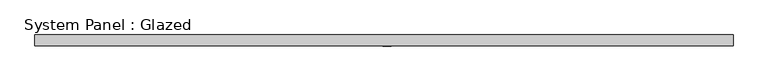
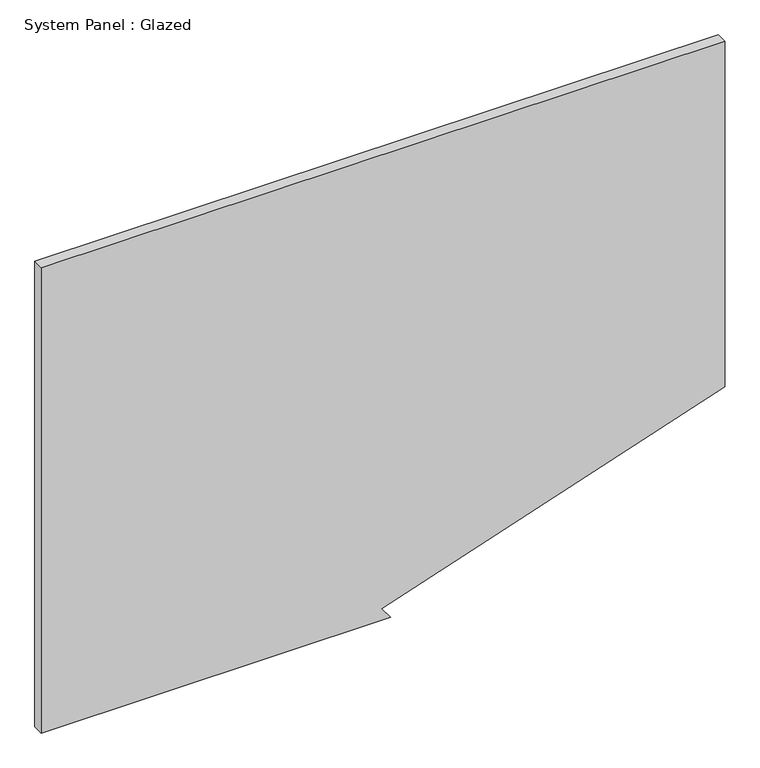
"""IFC4 building model written with IfcOpenShell, lengths in millimetres: plate geometry, System Panel : Glazed."""

from ifc_helpers import new_model, si_unit, frame, origin, place, context, project, spatial, polyline, outline, extrude, source, transform, mapped, element, save


def system_panel_glazed_3c16f4b8(model_context):
    return source(origin(), model_context, "Body", "SweptSolid", [
        extrude(outline(polyline([(0.0, -803.275), (0.0, 17.2127692), (28.4913894, -2.867694), (297.2056207, 803.275), (1155.7, 803.275), (1155.7, -803.275), (0.0, -803.275)])), frame((0.0, -44.45, 0.0), z_axis=(0.0, 1.0, 0.0), x_axis=(0.0, 0.0, 1.0)), (0.0, 0.0, 1.0), 25.4),
    ])


if __name__ == "__main__":
    model = new_model("IFC4")
    model_context = context("Model", 3, world=origin())
    ifc_project = project(units=[si_unit("LENGTHUNIT", "METRE", prefix="MILLI")], contexts=[model_context])
    site = spatial("IfcSite", under=ifc_project)
    building = spatial("IfcBuilding", under=site)
    placement = place(None, origin())
    system_panel_glazed_shape = system_panel_glazed_3c16f4b8(model_context)
    element("IfcPlate", 1, ObjectType="System Panel : Glazed", at=placement, inside=building, context=model_context, shape_type="MappedRepresentation", body=[
        mapped(system_panel_glazed_shape, transform((0.0, 0.0, 0.0), x_axis=(1.0, 0.0, 0.0), y_axis=(0.0, 1.0, 0.0), z_axis=(0.0, 0.0, 1.0))),
    ])
    save(model, "model.ifc")

# Revit data of these elements
# Element 1 (IfcPlate, "System Panel : Glazed")
#   Materials on its faces: "Glass"
# Materials
#   "Glass": class "Glass", colour RGB 0 128 192, transparency 0.75
